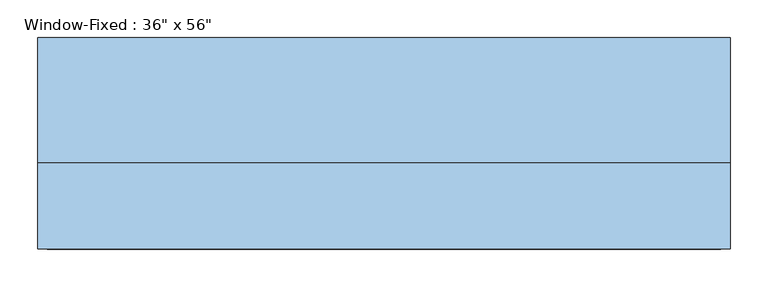
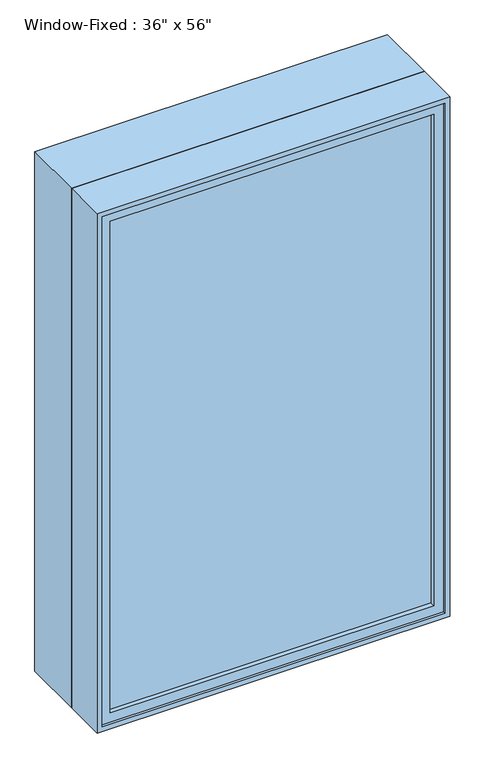
"""IFC4 building model written with IfcOpenShell, lengths in millimetres: window geometry."""

import ifcopenshell
import ifcopenshell.guid

model = None  # the IFC model being written
_history = None  # IfcOwnerHistory: only IFC2X3 demands one
_inside = {}  # id of a spatial element -> (the spatial element, [elements in it])
_under = {}  # id of a project, library or spatial element -> (it, [spatial elements below it])
_declared = {}  # id of a project -> (the project, [libraries it declares])
_typed = {}  # id of a type object -> (the type object, [elements of that type])
_made_of = {}  # id of a material, layer set ... -> (it, [elements and type objects made of it])


def new_model(schema):
    """Start an empty IFC model of exactly this schema.

    Asked for "IFC4X3", IfcOpenShell would pick the latest addendum, in which some entities
    have other attributes; the version numbers below select the first issue.
    IFC2X3 requires an IfcOwnerHistory on every rooted entity: one is made here for all.
    """
    global model, _history
    if schema == "IFC4X3":
        model = ifcopenshell.file(schema_version=(4, 3, 0, 0))
    else:
        model = ifcopenshell.file(schema=schema)
    _inside.clear()
    _under.clear()
    _declared.clear()
    _typed.clear()
    _made_of.clear()
    _history = None
    if model.schema == "IFC2X3":
        org = make("IfcOrganization", Name="unknown")
        user = make(
            "IfcPersonAndOrganization",
            ThePerson=make("IfcPerson", FamilyName="unknown"),
            TheOrganization=org,
        )
        app = make(
            "IfcApplication",
            ApplicationDeveloper=org,
            Version="unknown",
            ApplicationFullName="unknown",
            ApplicationIdentifier="unknown",
        )
        _history = make(
            "IfcOwnerHistory",
            OwningUser=user,
            OwningApplication=app,
            ChangeAction="ADDED",
            CreationDate=0,
        )
    return model


def make(cls, **values):
    """One entity of the class cls with the attributes given. An attribute that is None is left unset."""
    return model.create_entity(
        cls, **{name: value for name, value in values.items() if value is not None}
    )


def rooted(cls, **values):
    """An entity with a GlobalId (a new one), such as an element, a storey or a relation."""
    return make(cls, GlobalId=ifcopenshell.guid.new(), OwnerHistory=_history, **values)


def si_unit(unit_type, name, prefix=None):
    """IfcSIUnit, for example si_unit("LENGTHUNIT", "METRE", prefix="MILLI")."""
    return make("IfcSIUnit", UnitType=unit_type, Prefix=prefix, Name=name)


def assignment(units):
    """IfcUnitAssignment: the units of a project."""
    return None if units is None else make("IfcUnitAssignment", Units=units)


def point(xyz):
    """IfcCartesianPoint."""
    return None if xyz is None else make("IfcCartesianPoint", Coordinates=xyz)


def direction(xyz):
    """IfcDirection."""
    return None if xyz is None else make("IfcDirection", DirectionRatios=xyz)


def frame(location, z_axis=None, x_axis=None):
    """IfcAxis2Placement3D, a coordinate frame: its origin and axes. An axis left out is left unset."""
    return make(
        "IfcAxis2Placement3D",
        Location=point(location),
        Axis=direction(z_axis),
        RefDirection=direction(x_axis),
    )


def origin():
    """The frame at (0, 0, 0) with its axes left unset."""
    return frame((0.0, 0.0, 0.0))


def place(relative_to, where):
    """IfcLocalPlacement: puts the frame where relative to a parent placement (None: the world)."""
    return make(
        "IfcLocalPlacement", PlacementRelTo=relative_to, RelativePlacement=where
    )


def context(
    kind, dimensions, precision=None, world=None, true_north=None, identifier=None
):
    """IfcGeometricRepresentationContext, for example the 3D "Model" context."""
    return make(
        "IfcGeometricRepresentationContext",
        ContextIdentifier=identifier,
        ContextType=kind,
        CoordinateSpaceDimension=dimensions,
        Precision=precision,
        WorldCoordinateSystem=world,
        TrueNorth=true_north,
    )


def project(units=None, contexts=None):
    """IfcProject with its units and contexts."""
    return rooted(
        "IfcProject",
        Name="project",
        RepresentationContexts=contexts,
        UnitsInContext=assignment(units),
    )


def spatial(cls, under=None, at=None, **own):
    """A site, building, storey or space (cls), placed at a placement, below another one or the project."""
    s = rooted(cls, ObjectPlacement=at, **own)
    if under is not None:
        _under.setdefault(under.id(), (under, []))[1].append(s)
    return s


def polyline(points):
    """IfcPolyline through the points."""
    return make("IfcPolyline", Points=[point(p) for p in points])


def outline(outer, holes=None, kind="AREA"):
    """IfcArbitraryClosedProfileDef: a profile drawn as a closed curve; with holes, ...WithVoids."""
    if holes is None:
        return make("IfcArbitraryClosedProfileDef", ProfileType=kind, OuterCurve=outer)
    return make(
        "IfcArbitraryProfileDefWithVoids",
        ProfileType=kind,
        OuterCurve=outer,
        InnerCurves=holes,
    )


def extrude(swept, where, along, depth):
    """IfcExtrudedAreaSolid: the profile swept, set in the frame where, extruded along a direction by depth."""
    return make(
        "IfcExtrudedAreaSolid",
        SweptArea=swept,
        Position=where,
        ExtrudedDirection=direction(along),
        Depth=depth,
    )


def faces_of(points, faces, orient=None, outer=None):
    """IfcFace entities. A face is a list of loops; a loop is a list of indices into points, from 0.

    orient and outer hold one flag for each loop. By default every Orientation is true, the
    first loop of a face is its IfcFaceOuterBound and the others are IfcFaceBound.
    """
    made = []
    for i, loops in enumerate(faces):
        bounds = []
        for j, loop in enumerate(loops):
            is_outer = j == 0 if outer is None else outer[i][j]
            bounds.append(
                make(
                    "IfcFaceOuterBound" if is_outer else "IfcFaceBound",
                    Bound=make("IfcPolyLoop", Polygon=[points[k] for k in loop]),
                    Orientation=True if orient is None else orient[i][j],
                )
            )
        made.append(make("IfcFace", Bounds=bounds))
    return made


def faceted_brep(points, faces, orient=None, outer=None, voids=None):
    """IfcFacetedBrep: a solid bounded by flat faces; with voids (closed shells), ...WithVoids."""
    shared = [point(p) for p in points]
    hull = make("IfcClosedShell", CfsFaces=faces_of(shared, faces, orient, outer))
    if voids is None:
        return make("IfcFacetedBrep", Outer=hull)
    return make(
        "IfcFacetedBrepWithVoids",
        Outer=hull,
        Voids=[
            make(cls, CfsFaces=faces_of(shared, fs, o, b)) for cls, fs, o, b in voids
        ],
    )


def shape(context_of_items, identifier, shape_type, items):
    """IfcShapeRepresentation: the items that make up one representation, for example the "Body"."""
    return make(
        "IfcShapeRepresentation",
        ContextOfItems=context_of_items,
        RepresentationIdentifier=identifier,
        RepresentationType=shape_type,
        Items=items,
    )


def source(mapping_origin, context_of_items, identifier, shape_type, items):
    """IfcRepresentationMap: a shape defined once, which mapped items show again and again."""
    return make(
        "IfcRepresentationMap",
        MappingOrigin=mapping_origin,
        MappedRepresentation=shape(context_of_items, identifier, shape_type, items),
    )


def transform(
    local_origin,
    x_axis=None,
    y_axis=None,
    z_axis=None,
    scale=None,
    scale2=None,
    scale3=None,
    uniform=True,
):
    """IfcCartesianTransformationOperator3D, or its non-uniform kind. x_axis, y_axis, z_axis: its Axis1, 2, 3."""
    if uniform:
        return make(
            "IfcCartesianTransformationOperator3D",
            Axis1=direction(x_axis),
            Axis2=direction(y_axis),
            LocalOrigin=point(local_origin),
            Scale=scale,
            Axis3=direction(z_axis),
        )
    return make(
        "IfcCartesianTransformationOperator3DnonUniform",
        Axis1=direction(x_axis),
        Axis2=direction(y_axis),
        LocalOrigin=point(local_origin),
        Scale=scale,
        Axis3=direction(z_axis),
        Scale2=scale2,
        Scale3=scale3,
    )


def mapped(mapping_source, mapping_target):
    """IfcMappedItem: shows the shape of a source again, moved by a transform."""
    return make(
        "IfcMappedItem", MappingSource=mapping_source, MappingTarget=mapping_target
    )


def made_of(thing, what):
    """Note that an element or type object is made of a material, layer set ...; save() writes the relation."""
    if what is not None:
        _made_of.setdefault(what.id(), (what, []))[1].append(thing)
    return thing


def element(
    cls,
    number,
    at=None,
    inside=None,
    cuts=None,
    type_object=None,
    material=None,
    context=None,
    identifier="Body",
    shape_type=None,
    held_by="IfcProductDefinitionShape",
    body=None,
    shapes=None,
    **own,
):
    """One element of the class cls, such as IfcWall. Its Tag is "e" and its number.

    at: its placement. inside: the storey or other place that contains it. cuts: it is an
    opening in that element (IfcRelVoidsElement). A single representation is given by context,
    identifier, shape_type and body (its items); several are given by shapes. held_by: the class
    of the entity that holds the representations. save() writes the other relations.
    """
    e = rooted(cls, Tag="e%d" % number, ObjectPlacement=at, **own)
    if body is not None:
        shapes = [shape(context, identifier, shape_type, body)]
    if shapes is not None:
        e.Representation = make(held_by, Representations=shapes)
    if inside is not None:
        _inside.setdefault(inside.id(), (inside, []))[1].append(e)
    if cuts is not None:
        rooted(
            "IfcRelVoidsElement", RelatingBuildingElement=cuts, RelatedOpeningElement=e
        )
    if type_object is not None:
        _typed.setdefault(type_object.id(), (type_object, []))[1].append(e)
    return made_of(e, material)


def aggregate(whole, parts):
    """IfcRelAggregates: a whole, such as a stair, and the parts it consists of."""
    return rooted("IfcRelAggregates", RelatingObject=whole, RelatedObjects=parts)


def save(model, path):
    """Write the relations noted so far, then the file.

    IfcRelAggregates (storeys below a building ...), IfcRelContainedInSpatialStructure (elements
    in a storey), IfcRelDefinesByType, IfcRelAssociatesMaterial and IfcRelDeclares: one each for
    every whole, place, type object, material and project.
    """
    for whole, parts in _under.values():
        aggregate(whole, parts)
    for where, things in _inside.values():
        rooted(
            "IfcRelContainedInSpatialStructure",
            RelatedElements=things,
            RelatingStructure=where,
        )
    for kind, things in _typed.values():
        rooted("IfcRelDefinesByType", RelatedObjects=things, RelatingType=kind)
    for what, things in _made_of.values():
        rooted("IfcRelAssociatesMaterial", RelatedObjects=things, RelatingMaterial=what)
    for by, libraries in _declared.values():
        rooted("IfcRelDeclares", RelatingContext=by, RelatedDefinitions=libraries)
    model.write(path)


def window_f3e63972(model_context):
    return source(origin(), model_context, "Body", "SolidModel", [
        extrude(outline(polyline([(419.1, -104.775), (-419.1, -104.775), (-419.1, -98.425), (419.1, -98.425), (419.1, -104.775)])), frame((0.0, 0.0, 952.5), z_axis=(0.0, 0.0, 1.0), x_axis=(1.0, 0.0, 0.0)), (0.0, 0.0, 1.0), 1346.2),
        extrude(outline(polyline([(-419.1, -85.725), (419.1, -85.725), (419.1, -92.075), (-419.1, -92.075), (-419.1, -85.725)])), frame((0.0, 0.0, 952.5), z_axis=(0.0, 0.0, 1.0), x_axis=(1.0, 0.0, 0.0)), (0.0, 0.0, 1.0), 1346.2),
        extrude(outline(polyline([(927.1, -444.5), (927.1, 444.5), (2324.1, 444.5), (2324.1, -444.5), (927.1, -444.5)]), holes=[polyline([(952.5, 419.1), (952.5, -419.1), (2298.7, -419.1), (2298.7, 419.1), (952.5, 419.1)])]), frame((0.0, -117.475, 0.0), z_axis=(0.0, 1.0, 0.0), x_axis=(0.0, 0.0, 1.0)), (0.0, 0.0, 1.0), 44.45),
        extrude(outline(polyline([(2336.8, -457.2), (914.4, -457.2), (914.4, 457.2), (2336.8, 457.2), (2336.8, -457.2)]), holes=[polyline([(2324.1, 444.5), (927.1, 444.5), (927.1, -444.5), (2324.1, -444.5), (2324.1, 444.5)])]), frame((0.0, -9.525, 0.0), z_axis=(0.0, 1.0, 0.0), x_axis=(0.0, 0.0, 1.0)), (0.0, 0.0, 1.0), 165.1),
        faceted_brep([(457.2, -9.525, 2336.8), (-457.2, -9.525, 2336.8), (-457.2, -123.825, 2336.8), (457.2, -123.825, 2336.8), (-457.2, -9.525, 914.4), (-457.2, -123.825, 914.4), (457.2, -9.525, 914.4), (457.2, -123.825, 914.4), (425.45, -9.525, 2305.05), (-425.45, -9.525, 2305.05), (-425.45, -9.525, 946.15), (425.45, -9.525, 946.15), (-444.5, -123.825, 2324.1), (444.5, -123.825, 2324.1), (444.5, -123.825, 927.1), (-444.5, -123.825, 927.1), (425.45, -73.025, 2305.05), (-425.45, -73.025, 2305.05), (-444.5, -73.025, 2324.1), (444.5, -73.025, 2324.1), (-425.45, -73.025, 946.15), (-444.5, -73.025, 927.1), (425.45, -73.025, 946.15), (444.5, -73.025, 927.1)], [[[0, 1, 2, 3]], [[1, 4, 5, 2]], [[4, 6, 7, 5]], [[1, 0, 6, 4], [8, 9, 10, 11]], [[6, 0, 3, 7]], [[3, 2, 5, 7], [12, 13, 14, 15]], [[16, 17, 9, 8]], [[13, 12, 18, 19]], [[17, 20, 10, 9]], [[12, 15, 21, 18]], [[20, 22, 11, 10]], [[15, 14, 23, 21]], [[22, 16, 8, 11]], [[19, 18, 21, 23], [17, 16, 22, 20]], [[14, 13, 19, 23]]]),
    ])


if __name__ == "__main__":
    model = new_model("IFC4")
    model_context = context("Model", 3, world=origin())
    ifc_project = project(units=[si_unit("LENGTHUNIT", "METRE", prefix="MILLI")], contexts=[model_context])
    site = spatial("IfcSite", under=ifc_project)
    building = spatial("IfcBuilding", under=site)
    placement = place(None, origin())
    window_shape = window_f3e63972(model_context)
    element("IfcWindow", 1, ObjectType="Window-Fixed : 36\" x 56\"", at=placement, inside=building, context=model_context, shape_type="MappedRepresentation", body=[
        mapped(window_shape, transform((0.0, 0.0, 0.0), x_axis=(1.0, 0.0, 0.0), y_axis=(0.0, 1.0, 0.0), z_axis=(0.0, 0.0, 1.0))),
    ])
    save(model, "model.ifc")

# Revit data of these elements
# Type "Window-Fixed : 36\" x 56\""
#   Type Mark = "22"
#   Fire Rating = "0.5h"
#   Assembly Code = "B2020100"
#   Analytic Construction = "Double glazing - domestic"
#   Window Inset [instance default] = 0' - 0"
#   Wall Thickness [instance default] = 0' - 6"
#   Visual Light Transmittance = 0.81
#   Thermal Resistance (R) = 1.8146 (h·ft²·°F)/BTU
#   Solar Heat Gain Coefficient = 0.76
#   Rough Width = 3' - 0 1/2"
#   Rough Height = 4' - 8 1/2"
#   Interior Wall Closure [instance default] = 0' - 2 1/4"
#   Height = 4' - 8"
#   Heat Transfer Coefficient (U) = 0.5511 BTU/(h·ft²·°F)
#   Frame Extension [instance default] = 0' - 0 1/4"
#   Exterior Wall Closure [instance default] = 0' - 1 1/4"
#   Extension Jamb [instance default] = 0' - 2 1/4"
#   Default Sill Height = 3' - 0"
#   Width = 3' - 0"
#   Muntin Visibility = yes
#   Interior Trim Visibility [instance default] = yes
#   Exterior Trim Visibility [instance default] = yes
#   Extension Jamb Visibility [instance default] = yes
#   Muntin Pattern = Muntin Pattern_2x2 : Muntin Pattern_2x2
#   Interior Trim Material = Wood - Stained
#   Interior Trim = Trim-Window-Interior-Flat : Picture Frame
#   Interior Frame Material = Wood - Stained
#   Glass Panel Material = Glass
#   Exterior Trim Material = Clad - White
#   Exterior Trim = Trim-Window-Exterior-Flat : with Sill
#   Exterior Frame Material = Clad - White
#   Wall Closure = (empty or 0)
# Element 1 (IfcWindow, "Window-Fixed : 36\" x 56\"")
#   Window Inset = 0' - 2"
#   Wall Thickness = 1' - 0 1/4"
#   Exterior Wall Closure = 0' - 5 1/2"
#   Extension Jamb = 0' - 6 1/2"
#   Exterior Trim Visibility = no
#   Materials on its faces: "Wood - Stained", "Glass", "Clad - White"
# Materials
#   "Wood - Stained": class "Wood", colour RGB 224 178 126, transparency 0, Cost = 0
#   "Glass": class "Glass", colour RGB 0 128 192, transparency 0.75, Description = "Soda Lime Glass", Cost = 0
#   "Clad - White": class "Wood", colour RGB 242 242 238, transparency 0, Cost = 0
